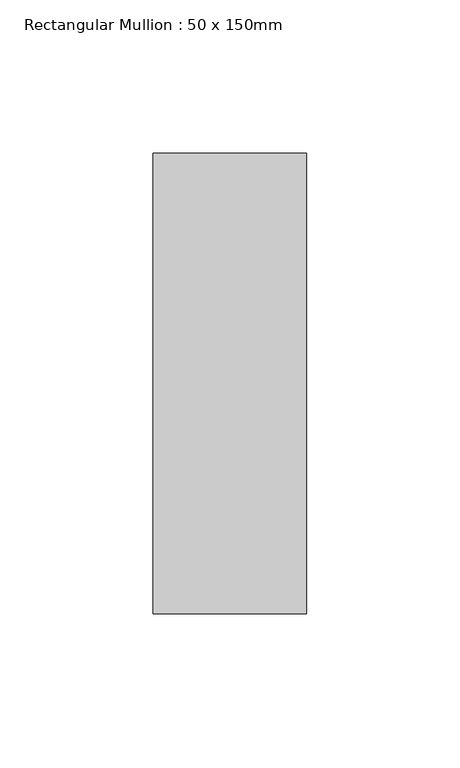
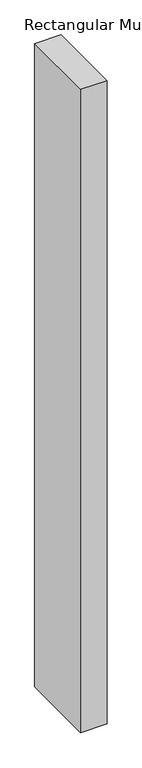
"""IFC4 building model written with IfcOpenShell, lengths in millimetres: member geometry, Rectangular Mullion : 50 x 150mm."""

import ifcopenshell
import ifcopenshell.guid

model = None  # the IFC model being written
_history = None  # IfcOwnerHistory: only IFC2X3 demands one
_inside = {}  # id of a spatial element -> (the spatial element, [elements in it])
_under = {}  # id of a project, library or spatial element -> (it, [spatial elements below it])
_declared = {}  # id of a project -> (the project, [libraries it declares])
_typed = {}  # id of a type object -> (the type object, [elements of that type])
_made_of = {}  # id of a material, layer set ... -> (it, [elements and type objects made of it])


def new_model(schema):
    """Start an empty IFC model of exactly this schema.

    Asked for "IFC4X3", IfcOpenShell would pick the latest addendum, in which some entities
    have other attributes; the version numbers below select the first issue.
    IFC2X3 requires an IfcOwnerHistory on every rooted entity: one is made here for all.
    """
    global model, _history
    if schema == "IFC4X3":
        model = ifcopenshell.file(schema_version=(4, 3, 0, 0))
    else:
        model = ifcopenshell.file(schema=schema)
    _inside.clear()
    _under.clear()
    _declared.clear()
    _typed.clear()
    _made_of.clear()
    _history = None
    if model.schema == "IFC2X3":
        org = make("IfcOrganization", Name="unknown")
        user = make(
            "IfcPersonAndOrganization",
            ThePerson=make("IfcPerson", FamilyName="unknown"),
            TheOrganization=org,
        )
        app = make(
            "IfcApplication",
            ApplicationDeveloper=org,
            Version="unknown",
            ApplicationFullName="unknown",
            ApplicationIdentifier="unknown",
        )
        _history = make(
            "IfcOwnerHistory",
            OwningUser=user,
            OwningApplication=app,
            ChangeAction="ADDED",
            CreationDate=0,
        )
    return model


def make(cls, **values):
    """One entity of the class cls with the attributes given. An attribute that is None is left unset."""
    return model.create_entity(
        cls, **{name: value for name, value in values.items() if value is not None}
    )


def rooted(cls, **values):
    """An entity with a GlobalId (a new one), such as an element, a storey or a relation."""
    return make(cls, GlobalId=ifcopenshell.guid.new(), OwnerHistory=_history, **values)


def si_unit(unit_type, name, prefix=None):
    """IfcSIUnit, for example si_unit("LENGTHUNIT", "METRE", prefix="MILLI")."""
    return make("IfcSIUnit", UnitType=unit_type, Prefix=prefix, Name=name)


def assignment(units):
    """IfcUnitAssignment: the units of a project."""
    return None if units is None else make("IfcUnitAssignment", Units=units)


def point(xyz):
    """IfcCartesianPoint."""
    return None if xyz is None else make("IfcCartesianPoint", Coordinates=xyz)


def direction(xyz):
    """IfcDirection."""
    return None if xyz is None else make("IfcDirection", DirectionRatios=xyz)


def frame(location, z_axis=None, x_axis=None):
    """IfcAxis2Placement3D, a coordinate frame: its origin and axes. An axis left out is left unset."""
    return make(
        "IfcAxis2Placement3D",
        Location=point(location),
        Axis=direction(z_axis),
        RefDirection=direction(x_axis),
    )


def origin():
    """The frame at (0, 0, 0) with its axes left unset."""
    return frame((0.0, 0.0, 0.0))


def place(relative_to, where):
    """IfcLocalPlacement: puts the frame where relative to a parent placement (None: the world)."""
    return make(
        "IfcLocalPlacement", PlacementRelTo=relative_to, RelativePlacement=where
    )


def context(
    kind, dimensions, precision=None, world=None, true_north=None, identifier=None
):
    """IfcGeometricRepresentationContext, for example the 3D "Model" context."""
    return make(
        "IfcGeometricRepresentationContext",
        ContextIdentifier=identifier,
        ContextType=kind,
        CoordinateSpaceDimension=dimensions,
        Precision=precision,
        WorldCoordinateSystem=world,
        TrueNorth=true_north,
    )


def project(units=None, contexts=None):
    """IfcProject with its units and contexts."""
    return rooted(
        "IfcProject",
        Name="project",
        RepresentationContexts=contexts,
        UnitsInContext=assignment(units),
    )


def spatial(cls, under=None, at=None, **own):
    """A site, building, storey or space (cls), placed at a placement, below another one or the project."""
    s = rooted(cls, ObjectPlacement=at, **own)
    if under is not None:
        _under.setdefault(under.id(), (under, []))[1].append(s)
    return s


def polyline(points):
    """IfcPolyline through the points."""
    return make("IfcPolyline", Points=[point(p) for p in points])


def outline(outer, holes=None, kind="AREA"):
    """IfcArbitraryClosedProfileDef: a profile drawn as a closed curve; with holes, ...WithVoids."""
    if holes is None:
        return make("IfcArbitraryClosedProfileDef", ProfileType=kind, OuterCurve=outer)
    return make(
        "IfcArbitraryProfileDefWithVoids",
        ProfileType=kind,
        OuterCurve=outer,
        InnerCurves=holes,
    )


def extrude(swept, where, along, depth):
    """IfcExtrudedAreaSolid: the profile swept, set in the frame where, extruded along a direction by depth."""
    return make(
        "IfcExtrudedAreaSolid",
        SweptArea=swept,
        Position=where,
        ExtrudedDirection=direction(along),
        Depth=depth,
    )


def shape(context_of_items, identifier, shape_type, items):
    """IfcShapeRepresentation: the items that make up one representation, for example the "Body"."""
    return make(
        "IfcShapeRepresentation",
        ContextOfItems=context_of_items,
        RepresentationIdentifier=identifier,
        RepresentationType=shape_type,
        Items=items,
    )


def source(mapping_origin, context_of_items, identifier, shape_type, items):
    """IfcRepresentationMap: a shape defined once, which mapped items show again and again."""
    return make(
        "IfcRepresentationMap",
        MappingOrigin=mapping_origin,
        MappedRepresentation=shape(context_of_items, identifier, shape_type, items),
    )


def transform(
    local_origin,
    x_axis=None,
    y_axis=None,
    z_axis=None,
    scale=None,
    scale2=None,
    scale3=None,
    uniform=True,
):
    """IfcCartesianTransformationOperator3D, or its non-uniform kind. x_axis, y_axis, z_axis: its Axis1, 2, 3."""
    if uniform:
        return make(
            "IfcCartesianTransformationOperator3D",
            Axis1=direction(x_axis),
            Axis2=direction(y_axis),
            LocalOrigin=point(local_origin),
            Scale=scale,
            Axis3=direction(z_axis),
        )
    return make(
        "IfcCartesianTransformationOperator3DnonUniform",
        Axis1=direction(x_axis),
        Axis2=direction(y_axis),
        LocalOrigin=point(local_origin),
        Scale=scale,
        Axis3=direction(z_axis),
        Scale2=scale2,
        Scale3=scale3,
    )


def mapped(mapping_source, mapping_target):
    """IfcMappedItem: shows the shape of a source again, moved by a transform."""
    return make(
        "IfcMappedItem", MappingSource=mapping_source, MappingTarget=mapping_target
    )


def made_of(thing, what):
    """Note that an element or type object is made of a material, layer set ...; save() writes the relation."""
    if what is not None:
        _made_of.setdefault(what.id(), (what, []))[1].append(thing)
    return thing


def element(
    cls,
    number,
    at=None,
    inside=None,
    cuts=None,
    type_object=None,
    material=None,
    context=None,
    identifier="Body",
    shape_type=None,
    held_by="IfcProductDefinitionShape",
    body=None,
    shapes=None,
    **own,
):
    """One element of the class cls, such as IfcWall. Its Tag is "e" and its number.

    at: its placement. inside: the storey or other place that contains it. cuts: it is an
    opening in that element (IfcRelVoidsElement). A single representation is given by context,
    identifier, shape_type and body (its items); several are given by shapes. held_by: the class
    of the entity that holds the representations. save() writes the other relations.
    """
    e = rooted(cls, Tag="e%d" % number, ObjectPlacement=at, **own)
    if body is not None:
        shapes = [shape(context, identifier, shape_type, body)]
    if shapes is not None:
        e.Representation = make(held_by, Representations=shapes)
    if inside is not None:
        _inside.setdefault(inside.id(), (inside, []))[1].append(e)
    if cuts is not None:
        rooted(
            "IfcRelVoidsElement", RelatingBuildingElement=cuts, RelatedOpeningElement=e
        )
    if type_object is not None:
        _typed.setdefault(type_object.id(), (type_object, []))[1].append(e)
    return made_of(e, material)


def aggregate(whole, parts):
    """IfcRelAggregates: a whole, such as a stair, and the parts it consists of."""
    return rooted("IfcRelAggregates", RelatingObject=whole, RelatedObjects=parts)


def save(model, path):
    """Write the relations noted so far, then the file.

    IfcRelAggregates (storeys below a building ...), IfcRelContainedInSpatialStructure (elements
    in a storey), IfcRelDefinesByType, IfcRelAssociatesMaterial and IfcRelDeclares: one each for
    every whole, place, type object, material and project.
    """
    for whole, parts in _under.values():
        aggregate(whole, parts)
    for where, things in _inside.values():
        rooted(
            "IfcRelContainedInSpatialStructure",
            RelatedElements=things,
            RelatingStructure=where,
        )
    for kind, things in _typed.values():
        rooted("IfcRelDefinesByType", RelatedObjects=things, RelatingType=kind)
    for what, things in _made_of.values():
        rooted("IfcRelAssociatesMaterial", RelatedObjects=things, RelatingMaterial=what)
    for by, libraries in _declared.values():
        rooted("IfcRelDeclares", RelatingContext=by, RelatedDefinitions=libraries)
    model.write(path)


def rectangular_mullion_50_x_150mm_87298841(model_context):
    return source(origin(), model_context, "Body", "SweptSolid", [
        extrude(outline(polyline([(0.0, 75.0), (0.0, -75.0), (-50.0, -75.0), (-50.0, 75.0), (0.0, 75.0)])), frame((0.0, 0.0, -1283.3333333), z_axis=(0.0, 0.0, 1.0), x_axis=(1.0, 0.0, 0.0)), (0.0, 0.0, 1.0), 1283.3333333),
    ])


if __name__ == "__main__":
    model = new_model("IFC4")
    model_context = context("Model", 3, world=origin())
    ifc_project = project(units=[si_unit("LENGTHUNIT", "METRE", prefix="MILLI")], contexts=[model_context])
    site = spatial("IfcSite", under=ifc_project)
    building = spatial("IfcBuilding", under=site)
    placement = place(None, origin())
    rectangular_mullion_50_x_150mm_shape = rectangular_mullion_50_x_150mm_87298841(model_context)
    element("IfcMember", 1, ObjectType="Rectangular Mullion : 50 x 150mm", at=placement, inside=building, context=model_context, shape_type="MappedRepresentation", body=[
        mapped(rectangular_mullion_50_x_150mm_shape, transform((0.0, 0.0, 0.0), x_axis=(1.0, 0.0, 0.0), y_axis=(0.0, 1.0, 0.0), z_axis=(0.0, 0.0, 1.0))),
    ])
    save(model, "model.ifc")

# Revit data of these elements
# Type "Rectangular Mullion : 50 x 150mm"
#   built-in parameter 1007304 = 0.492126 (stored number, unit not read)
#   built-in parameter 1007301 = 0.082021 (stored number, unit not read)
#   built-in parameter 1007300 = 0.082021 (stored number, unit not read)
# Element 1 (IfcMember, "Rectangular Mullion : 50 x 150mm")
#   Materials on its faces: "Metal - Aluminium"
# Materials
#   "Metal - Aluminium": class "Metal", colour RGB 247 247 247, transparency 0
